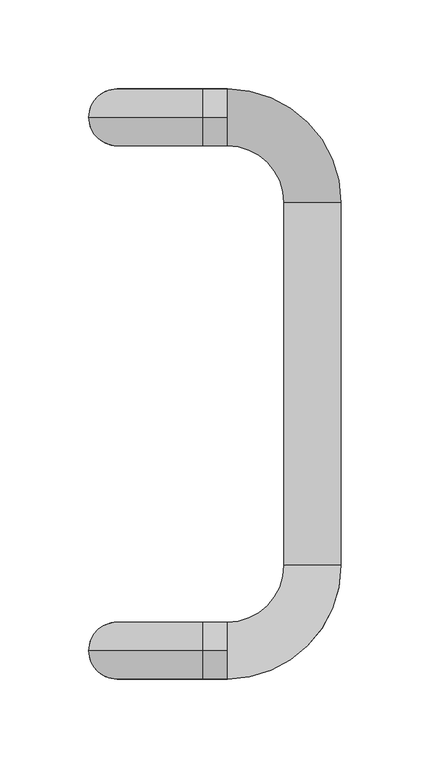
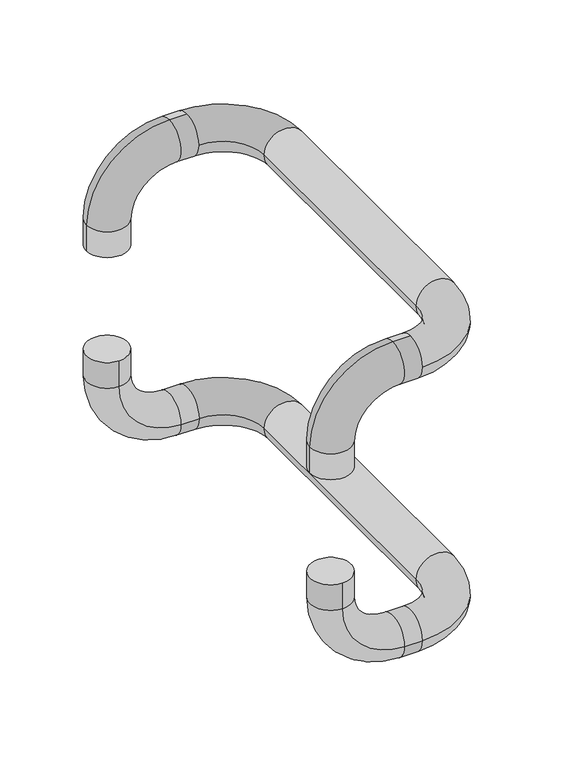
"""IFC4 building model written with IfcOpenShell, lengths in millimetres: proxy geometry, Architectural Hardware_HT7132_ASSA ABLOY_9402611AX26 : HT7132_9402611AX26."""

from ifc_helpers import new_model, si_unit, point, frame, origin, place, context, project, spatial, circle_curve, ellipse_curve, trimmed, source, transform, mapped, element, save
from ifc_brep_helpers import plane_surface, cylinder_surface, revolved_surface, advanced_brep


def specialty_equipment_07a0182d(model_context):
    return source(origin(), model_context, "Body", "AdvancedBrep", [
        advanced_brep(
        [(0.0, 166.0, -86.0), (0.0, 134.0, -86.0), (0.0, 134.0, -107.0), (0.0, 166.0, -107.0), (48.0, 134.0, -155.0), (48.0, 166.0, -155.0), (62.0, 134.0, -155.0), (62.0, 166.0, -155.0), (94.0, -102.0, -155.0), (126.0, -102.0, -155.0), (62.0, -166.0, -155.0), (62.0, -134.0, -155.0), (94.0, 102.0, -155.0), (126.0, 102.0, -155.0), (0.0, -166.0, -86.0), (0.0, -134.0, -86.0), (0.0, -166.0, -107.0), (0.0, -134.0, -107.0), (48.0, -166.0, -155.0), (48.0, -134.0, -155.0)],
        [
            (0, 1, circle_curve(frame((0.0, 150.0, -86.0), z_axis=(0.0, 0.0, 1.0), x_axis=(0.0, -1.0, 0.0)), 16.0)),
            (1, 0, circle_curve(frame((0.0, 150.0, -86.0), z_axis=(0.0, 0.0, 1.0), x_axis=(0.0, -1.0, 0.0)), 16.0)),
            (1, 2),
            (2, 3, circle_curve(frame((0.0, 150.0, -107.0), z_axis=(0.0, 0.0, 1.0), x_axis=(0.0, -1.0, 0.0)), 16.0)),
            (3, 0),
            (3, 2, circle_curve(frame((0.0, 150.0, -107.0), z_axis=(0.0, 0.0, 1.0), x_axis=(0.0, -1.0, 0.0)), 16.0)),
            (2, 4, circle_curve(frame((48.0, 134.0, -107.0), z_axis=(0.0, -1.0, 0.0), x_axis=(-1.0, 0.0, 0.0)), 48.0)),
            (4, 5, circle_curve(frame((48.0, 150.0, -155.0), z_axis=(-1.0, 0.0, 0.0), x_axis=(0.0, -1.0, 0.0)), 16.0)),
            (5, 3, circle_curve(frame((48.0, 166.0, -107.0), z_axis=(0.0, 1.0, 0.0), x_axis=(-1.0, 0.0, 0.0)), 48.0)),
            (5, 4, circle_curve(frame((48.0, 150.0, -155.0), z_axis=(-1.0, 0.0, 0.0), x_axis=(0.0, -1.0, 0.0)), 16.0)),
            (4, 6),
            (6, 7, circle_curve(frame((62.0, 150.0, -155.0), z_axis=(-1.0, 0.0, 0.0), x_axis=(0.0, -1.0, 0.0)), 16.0)),
            (7, 5),
            (7, 6, circle_curve(frame((62.0, 150.0, -155.0), z_axis=(-1.0, 0.0, 0.0), x_axis=(0.0, -1.0, 0.0)), 16.0)),
            (8, 9, circle_curve(frame((110.0, -102.0, -155.0), z_axis=(0.0, -1.0, 0.0), x_axis=(1.0, 0.0, 0.0)), 16.0)),
            (9, 10, circle_curve(frame((62.0, -102.0, -155.0), z_axis=(0.0, 0.0, -1.0), x_axis=(0.0, -1.0, 0.0)), 64.0)),
            (10, 11, circle_curve(frame((62.0, -150.0, -155.0), z_axis=(1.0, 0.0, 0.0), x_axis=(0.0, -1.0, 0.0)), 16.0)),
            (11, 8, circle_curve(frame((62.0, -102.0, -155.0), z_axis=(0.0, 0.0, 1.0), x_axis=(0.0, -1.0, 0.0)), 32.0)),
            (11, 10, circle_curve(frame((62.0, -150.0, -155.0), z_axis=(1.0, 0.0, 0.0), x_axis=(0.0, -1.0, 0.0)), 16.0)),
            (9, 8, circle_curve(frame((110.0, -102.0, -155.0), z_axis=(0.0, -1.0, 0.0), x_axis=(1.0, 0.0, 0.0)), 16.0)),
            (8, 12),
            (12, 13, circle_curve(frame((110.0, 102.0, -155.0), z_axis=(0.0, -1.0, 0.0), x_axis=(1.0, 0.0, 0.0)), 16.0)),
            (13, 9),
            (13, 12, circle_curve(frame((110.0, 102.0, -155.0), z_axis=(0.0, -1.0, 0.0), x_axis=(1.0, 0.0, 0.0)), 16.0)),
            (12, 6, circle_curve(frame((62.0, 102.0, -155.0), z_axis=(0.0, 0.0, 1.0), x_axis=(1.0, 0.0, 0.0)), 32.0)),
            (7, 13, circle_curve(frame((62.0, 102.0, -155.0), z_axis=(0.0, 0.0, -1.0), x_axis=(1.0, 0.0, 0.0)), 64.0)),
            (14, 15, circle_curve(frame((0.0, -150.0, -86.0), z_axis=(0.0, 0.0, 1.0), x_axis=(0.0, 1.0, 0.0)), 16.0)),
            (15, 14, circle_curve(frame((0.0, -150.0, -86.0), z_axis=(0.0, 0.0, 1.0), x_axis=(0.0, 1.0, 0.0)), 16.0)),
            (14, 16),
            (16, 17, circle_curve(frame((0.0, -150.0, -107.0), z_axis=(0.0, 0.0, 1.0), x_axis=(0.0, 1.0, 0.0)), 16.0)),
            (17, 15),
            (17, 16, circle_curve(frame((0.0, -150.0, -107.0), z_axis=(0.0, 0.0, 1.0), x_axis=(0.0, 1.0, 0.0)), 16.0)),
            (16, 18, circle_curve(frame((48.0, -166.0, -107.0), z_axis=(0.0, -1.0, 0.0), x_axis=(-1.0, 0.0, 0.0)), 48.0)),
            (18, 19, circle_curve(frame((48.0, -150.0, -155.0), z_axis=(-1.0, 0.0, 0.0), x_axis=(0.0, 1.0, 0.0)), 16.0)),
            (19, 17, circle_curve(frame((48.0, -134.0, -107.0), z_axis=(0.0, 1.0, 0.0), x_axis=(-1.0, 0.0, 0.0)), 48.0)),
            (19, 18, circle_curve(frame((48.0, -150.0, -155.0), z_axis=(-1.0, 0.0, 0.0), x_axis=(0.0, 1.0, 0.0)), 16.0)),
            (18, 10),
            (11, 19),
        ],
        [
            plane_surface(frame((0.0, 0.0, -86.0), z_axis=(0.0, 0.0, 1.0), x_axis=(0.0, -1.0, 0.0))),
            cylinder_surface(frame((0.0, 150.0, -86.0), z_axis=(0.0, 0.0, 1.0), x_axis=(0.0, -1.0, 0.0)), 16.0),
            revolved_surface(trimmed(ellipse_curve(frame((0.0, 150.0, -107.0), z_axis=(0.0, 0.0, -1.0), x_axis=(0.0, -1.0, 0.0)), 16.0, 16.0), [point((0.0, 166.0, -107.0))], [point((0.0, 134.0, -107.0))], True, "CARTESIAN"), (48.0, 0.0, -107.0), (0.0, 1.0, 0.0)),
            revolved_surface(trimmed(ellipse_curve(frame((0.0, 150.0, -107.0), z_axis=(0.0, 0.0, -1.0), x_axis=(0.0, -1.0, 0.0)), 16.0, 16.0), [point((0.0, 134.0, -107.0))], [point((0.0, 166.0, -107.0))], True, "CARTESIAN"), (48.0, 0.0, -107.0), (0.0, 1.0, 0.0)),
            cylinder_surface(frame((48.0, 150.0, -155.0), z_axis=(-1.0, 0.0, 0.0), x_axis=(0.0, -1.0, 0.0)), 16.0),
            revolved_surface(trimmed(ellipse_curve(frame((62.0, -150.0, -155.0), z_axis=(1.0, 0.0, 0.0), x_axis=(0.0, -1.0, 0.0)), 16.0, 16.0), [point((62.0, -166.0, -155.0))], [point((62.0, -134.0, -155.0))], True, "CARTESIAN"), (62.0, -102.0, -86.0), (0.0, 0.0, -1.0)),
            revolved_surface(trimmed(ellipse_curve(frame((62.0, -150.0, -155.0), z_axis=(1.0, 0.0, 0.0), x_axis=(0.0, -1.0, 0.0)), 16.0, 16.0), [point((62.0, -134.0, -155.0))], [point((62.0, -166.0, -155.0))], True, "CARTESIAN"), (62.0, -102.0, -86.0), (0.0, 0.0, -1.0)),
            cylinder_surface(frame((110.0, -102.0, -155.0), z_axis=(0.0, -1.0, 0.0), x_axis=(1.0, 0.0, 0.0)), 16.0),
            revolved_surface(trimmed(ellipse_curve(frame((110.0, 102.0, -155.0), z_axis=(0.0, 1.0, 0.0), x_axis=(1.0, 0.0, 0.0)), 16.0, 16.0), [point((126.0, 102.0, -155.0))], [point((94.0, 102.0, -155.0))], True, "CARTESIAN"), (62.0, 102.0, -86.0), (0.0, 0.0, -1.0)),
            revolved_surface(trimmed(ellipse_curve(frame((110.0, 102.0, -155.0), z_axis=(0.0, 1.0, 0.0), x_axis=(1.0, 0.0, 0.0)), 16.0, 16.0), [point((94.0, 102.0, -155.0))], [point((126.0, 102.0, -155.0))], True, "CARTESIAN"), (62.0, 102.0, -86.0), (0.0, 0.0, -1.0)),
            plane_surface(frame((0.0, 0.0, -86.0), z_axis=(0.0, 0.0, 1.0), x_axis=(0.0, 1.0, 0.0))),
            cylinder_surface(frame((0.0, -150.0, -86.0), z_axis=(0.0, 0.0, 1.0), x_axis=(0.0, 1.0, 0.0)), 16.0),
            revolved_surface(trimmed(ellipse_curve(frame((0.0, -150.0, -107.0), z_axis=(0.0, 0.0, -1.0), x_axis=(0.0, 1.0, 0.0)), 16.0, 16.0), [point((0.0, -134.0, -107.0))], [point((0.0, -166.0, -107.0))], True, "CARTESIAN"), (48.0, 0.0, -107.0), (0.0, 1.0, 0.0)),
            revolved_surface(trimmed(ellipse_curve(frame((0.0, -150.0, -107.0), z_axis=(0.0, 0.0, -1.0), x_axis=(0.0, 1.0, 0.0)), 16.0, 16.0), [point((0.0, -166.0, -107.0))], [point((0.0, -134.0, -107.0))], True, "CARTESIAN"), (48.0, 0.0, -107.0), (0.0, 1.0, 0.0)),
            cylinder_surface(frame((48.0, -150.0, -155.0), z_axis=(-1.0, 0.0, 0.0), x_axis=(0.0, 1.0, 0.0)), 16.0),
        ],
        [
            (0, [[1, 2]]),
            (1, [[3, 4, 5, -2]]),
            (1, [[-5, 6, -3, -1]]),
            (2, [[7, 8, 9, -4]]),
            (3, [[-9, 10, -7, -6]]),
            (4, [[11, 12, 13, -8]]),
            (4, [[-13, 14, -11, -10]]),
            (5, [[15, 16, 17, 18]]),
            (6, [[19, -16, 20, -18]]),
            (7, [[21, 22, 23, -15]]),
            (7, [[-23, 24, -21, -20]]),
            (8, [[25, -14, 26, -22]]),
            (9, [[-26, -12, -25, -24]]),
            (10, [[27, 28]]),
            (11, [[29, 30, 31, -27]]),
            (11, [[-31, 32, -29, -28]]),
            (12, [[33, 34, 35, -30]]),
            (13, [[-35, 36, -33, -32]]),
            (14, [[37, -19, 38, -34]]),
            (14, [[-38, -17, -37, -36]]),
        ],
    ),
        advanced_brep(
        [(94.0, -102.0, 69.0), (126.0, -102.0, 69.0), (62.0, -166.0, 69.0), (62.0, -150.0, 53.0), (62.0, -134.0, 69.0), (62.0, -150.0, 85.0), (94.0, 102.0, 69.0), (126.0, 102.0, 69.0), (62.0, 134.0, 69.0), (62.0, 150.0, 53.0), (62.0, 166.0, 69.0), (62.0, 150.0, 85.0), (-16.0, -150.0, 0.0), (16.0, -150.0, 0.0), (16.0, -150.0, 21.0), (-16.0, -150.0, 21.0), (48.0, -150.0, 53.0), (48.0, -150.0, 85.0), (-16.0, 150.0, 0.0), (16.0, 150.0, 0.0), (-16.0, 150.0, 21.0), (16.0, 150.0, 21.0), (48.0, 150.0, 85.0), (48.0, 150.0, 53.0)],
        [
            (0, 1, circle_curve(frame((110.0, -102.0, 69.0), z_axis=(0.0, -1.0, 0.0), x_axis=(-1.0, 0.0, 0.0)), 16.0)),
            (1, 2, circle_curve(frame((62.0, -102.0, 69.0), z_axis=(0.0, 0.0, -1.0), x_axis=(0.0, -1.0, 0.0)), 64.0)),
            (2, 3, circle_curve(frame((62.0, -150.0, 69.0), z_axis=(1.0, 0.0, 0.0), x_axis=(0.0, 1.0, 0.0)), 16.0)),
            (3, 4, circle_curve(frame((62.0, -150.0, 69.0), z_axis=(1.0, 0.0, 0.0), x_axis=(0.0, 1.0, 0.0)), 16.0)),
            (4, 0, circle_curve(frame((62.0, -102.0, 69.0), z_axis=(0.0, 0.0, 1.0), x_axis=(0.0, -1.0, 0.0)), 32.0)),
            (4, 5, circle_curve(frame((62.0, -150.0, 69.0), z_axis=(1.0, 0.0, 0.0), x_axis=(0.0, 1.0, 0.0)), 16.0)),
            (5, 2, circle_curve(frame((62.0, -150.0, 69.0), z_axis=(1.0, 0.0, 0.0), x_axis=(0.0, 1.0, 0.0)), 16.0)),
            (1, 0, circle_curve(frame((110.0, -102.0, 69.0), z_axis=(0.0, -1.0, 0.0), x_axis=(-1.0, 0.0, 0.0)), 16.0)),
            (0, 6),
            (6, 7, circle_curve(frame((110.0, 102.0, 69.0), z_axis=(0.0, -1.0, 0.0), x_axis=(-1.0, 0.0, 0.0)), 16.0)),
            (7, 1),
            (7, 6, circle_curve(frame((110.0, 102.0, 69.0), z_axis=(0.0, -1.0, 0.0), x_axis=(-1.0, 0.0, 0.0)), 16.0)),
            (6, 8, circle_curve(frame((62.0, 102.0, 69.0), z_axis=(0.0, 0.0, 1.0), x_axis=(1.0, 0.0, 0.0)), 32.0)),
            (8, 9, circle_curve(frame((62.0, 150.0, 69.0), z_axis=(1.0, 0.0, 0.0), x_axis=(0.0, -1.0, 0.0)), 16.0)),
            (9, 10, circle_curve(frame((62.0, 150.0, 69.0), z_axis=(1.0, 0.0, 0.0), x_axis=(0.0, -1.0, 0.0)), 16.0)),
            (10, 7, circle_curve(frame((62.0, 102.0, 69.0), z_axis=(0.0, 0.0, -1.0), x_axis=(1.0, 0.0, 0.0)), 64.0)),
            (10, 11, circle_curve(frame((62.0, 150.0, 69.0), z_axis=(1.0, 0.0, 0.0), x_axis=(0.0, -1.0, 0.0)), 16.0)),
            (11, 8, circle_curve(frame((62.0, 150.0, 69.0), z_axis=(1.0, 0.0, 0.0), x_axis=(0.0, -1.0, 0.0)), 16.0)),
            (12, 13, circle_curve(frame((0.0, -150.0, 0.0), z_axis=(0.0, 0.0, -1.0), x_axis=(1.0, 0.0, 0.0)), 16.0)),
            (13, 12, circle_curve(frame((0.0, -150.0, 0.0), z_axis=(0.0, 0.0, -1.0), x_axis=(1.0, 0.0, 0.0)), 16.0)),
            (13, 14),
            (14, 15, circle_curve(frame((0.0, -150.0, 21.0), z_axis=(0.0, 0.0, -1.0), x_axis=(1.0, 0.0, 0.0)), 16.0)),
            (15, 12),
            (15, 14, circle_curve(frame((0.0, -150.0, 21.0), z_axis=(0.0, 0.0, -1.0), x_axis=(1.0, 0.0, 0.0)), 16.0)),
            (14, 16, circle_curve(frame((48.0, -150.0, 21.0), z_axis=(0.0, 1.0, 0.0), x_axis=(-1.0, 0.0, 0.0)), 32.0)),
            (16, 17, circle_curve(frame((48.0, -150.0, 69.0), z_axis=(-1.0, 0.0, 0.0), x_axis=(0.0, 0.0, -1.0)), 16.0)),
            (17, 15, circle_curve(frame((48.0, -150.0, 21.0), z_axis=(0.0, -1.0, 0.0), x_axis=(-1.0, 0.0, 0.0)), 64.0)),
            (17, 16, circle_curve(frame((48.0, -150.0, 69.0), z_axis=(-1.0, 0.0, 0.0), x_axis=(0.0, 0.0, -1.0)), 16.0)),
            (16, 3),
            (5, 17),
            (18, 19, circle_curve(frame((0.0, 150.0, 0.0), z_axis=(0.0, 0.0, -1.0), x_axis=(1.0, 0.0, 0.0)), 16.0)),
            (19, 18, circle_curve(frame((0.0, 150.0, 0.0), z_axis=(0.0, 0.0, -1.0), x_axis=(1.0, 0.0, 0.0)), 16.0)),
            (18, 20),
            (20, 21, circle_curve(frame((0.0, 150.0, 21.0), z_axis=(0.0, 0.0, -1.0), x_axis=(1.0, 0.0, 0.0)), 16.0)),
            (21, 19),
            (21, 20, circle_curve(frame((0.0, 150.0, 21.0), z_axis=(0.0, 0.0, -1.0), x_axis=(1.0, 0.0, 0.0)), 16.0)),
            (20, 22, circle_curve(frame((48.0, 150.0, 21.0), z_axis=(0.0, 1.0, 0.0), x_axis=(-1.0, 0.0, 0.0)), 64.0)),
            (22, 23, circle_curve(frame((48.0, 150.0, 69.0), z_axis=(-1.0, 0.0, 0.0), x_axis=(0.0, 0.0, -1.0)), 16.0)),
            (23, 21, circle_curve(frame((48.0, 150.0, 21.0), z_axis=(0.0, -1.0, 0.0), x_axis=(-1.0, 0.0, 0.0)), 32.0)),
            (23, 22, circle_curve(frame((48.0, 150.0, 69.0), z_axis=(-1.0, 0.0, 0.0), x_axis=(0.0, 0.0, -1.0)), 16.0)),
            (22, 11),
            (9, 23),
        ],
        [
            revolved_surface(trimmed(ellipse_curve(frame((62.0, -150.0, 69.0), z_axis=(1.0, 0.0, 0.0), x_axis=(0.0, 1.0, 0.0)), 16.0, 16.0), [point((62.0, -166.0, 69.0))], [point((62.0, -134.0, 69.0))], True, "CARTESIAN"), (62.0, -102.0, 0.0), (0.0, 0.0, -1.0)),
            revolved_surface(trimmed(ellipse_curve(frame((62.0, -150.0, 69.0), z_axis=(1.0, 0.0, 0.0), x_axis=(0.0, 1.0, 0.0)), 16.0, 16.0), [point((62.0, -134.0, 69.0))], [point((62.0, -166.0, 69.0))], True, "CARTESIAN"), (62.0, -102.0, 0.0), (0.0, 0.0, -1.0)),
            cylinder_surface(frame((110.0, -102.0, 69.0), z_axis=(0.0, -1.0, 0.0), x_axis=(-1.0, 0.0, 0.0)), 16.0),
            revolved_surface(trimmed(ellipse_curve(frame((110.0, 102.0, 69.0), z_axis=(0.0, 1.0, 0.0), x_axis=(-1.0, 0.0, 0.0)), 16.0, 16.0), [point((126.0, 102.0, 69.0))], [point((94.0, 102.0, 69.0))], True, "CARTESIAN"), (62.0, 102.0, 0.0), (0.0, 0.0, -1.0)),
            revolved_surface(trimmed(ellipse_curve(frame((110.0, 102.0, 69.0), z_axis=(0.0, 1.0, 0.0), x_axis=(-1.0, 0.0, 0.0)), 16.0, 16.0), [point((94.0, 102.0, 69.0))], [point((126.0, 102.0, 69.0))], True, "CARTESIAN"), (62.0, 102.0, 0.0), (0.0, 0.0, -1.0)),
            plane_surface(frame((0.0, 0.0, 0.0), z_axis=(0.0, 0.0, -1.0), x_axis=(0.0, 1.0, 0.0))),
            cylinder_surface(frame((0.0, -150.0, 0.0), z_axis=(0.0, 0.0, -1.0), x_axis=(1.0, 0.0, 0.0)), 16.0),
            revolved_surface(trimmed(ellipse_curve(frame((0.0, -150.0, 21.0), z_axis=(0.0, 0.0, 1.0), x_axis=(1.0, 0.0, 0.0)), 16.0, 16.0), [point((-16.0, -150.0, 21.0))], [point((16.0, -150.0, 21.0))], True, "CARTESIAN"), (48.0, 0.0, 21.0), (0.0, -1.0, 0.0)),
            revolved_surface(trimmed(ellipse_curve(frame((0.0, -150.0, 21.0), z_axis=(0.0, 0.0, 1.0), x_axis=(1.0, 0.0, 0.0)), 16.0, 16.0), [point((16.0, -150.0, 21.0))], [point((-16.0, -150.0, 21.0))], True, "CARTESIAN"), (48.0, 0.0, 21.0), (0.0, -1.0, 0.0)),
            cylinder_surface(frame((48.0, -150.0, 69.0), z_axis=(-1.0, 0.0, 0.0), x_axis=(0.0, 0.0, -1.0)), 16.0),
            plane_surface(frame((0.0, 0.0, 0.0), z_axis=(0.0, 0.0, -1.0), x_axis=(0.0, -1.0, 0.0))),
            cylinder_surface(frame((0.0, 150.0, 0.0), z_axis=(0.0, 0.0, -1.0), x_axis=(1.0, 0.0, 0.0)), 16.0),
            revolved_surface(trimmed(ellipse_curve(frame((0.0, 150.0, 21.0), z_axis=(0.0, 0.0, 1.0), x_axis=(1.0, 0.0, 0.0)), 16.0, 16.0), [point((16.0, 150.0, 21.0))], [point((-16.0, 150.0, 21.0))], True, "CARTESIAN"), (48.0, 0.0, 21.0), (0.0, -1.0, 0.0)),
            revolved_surface(trimmed(ellipse_curve(frame((0.0, 150.0, 21.0), z_axis=(0.0, 0.0, 1.0), x_axis=(1.0, 0.0, 0.0)), 16.0, 16.0), [point((-16.0, 150.0, 21.0))], [point((16.0, 150.0, 21.0))], True, "CARTESIAN"), (48.0, 0.0, 21.0), (0.0, -1.0, 0.0)),
            cylinder_surface(frame((48.0, 150.0, 69.0), z_axis=(-1.0, 0.0, 0.0), x_axis=(0.0, 0.0, -1.0)), 16.0),
        ],
        [
            (0, [[1, 2, 3, 4, 5]]),
            (1, [[6, 7, -2, 8, -5]]),
            (2, [[9, 10, 11, -1]]),
            (2, [[-11, 12, -9, -8]]),
            (3, [[13, 14, 15, 16, -10]]),
            (4, [[-16, 17, 18, -13, -12]]),
            (5, [[19, 20]]),
            (6, [[21, 22, 23, -20]]),
            (6, [[-23, 24, -21, -19]]),
            (7, [[25, 26, 27, -22]]),
            (8, [[-27, 28, -25, -24]]),
            (9, [[29, -3, -7, 30, -26]]),
            (9, [[-30, -6, -4, -29, -28]]),
            (10, [[31, 32]]),
            (11, [[33, 34, 35, -31]]),
            (11, [[-35, 36, -33, -32]]),
            (12, [[37, 38, 39, -34]]),
            (13, [[-39, 40, -37, -36]]),
            (14, [[41, -17, -15, 42, -38]]),
            (14, [[-42, -14, -18, -41, -40]]),
        ],
    ),
    ])


if __name__ == "__main__":
    model = new_model("IFC4")
    model_context = context("Model", 3, world=origin())
    ifc_project = project(units=[si_unit("LENGTHUNIT", "METRE", prefix="MILLI")], contexts=[model_context])
    site = spatial("IfcSite", under=ifc_project)
    building = spatial("IfcBuilding", under=site)
    placement = place(None, origin())
    specialty_equipment_shape = specialty_equipment_07a0182d(model_context)
    element("IfcBuildingElementProxy", 1, Name="Architectural Hardware_HT7132_ASSA ABLOY_9402611AX26 : HT7132_9402611AX26", ObjectType="Architectural Hardware_HT7132_ASSA ABLOY_9402611AX26 : HT7132_9402611AX26", at=placement, inside=building, context=model_context, shape_type="MappedRepresentation", body=[
        mapped(specialty_equipment_shape, transform((0.0, 0.0, 0.0), x_axis=(1.0, 0.0, 0.0), y_axis=(0.0, 1.0, 0.0), z_axis=(0.0, 0.0, 1.0))),
    ])
    save(model, "model.ifc")

# Revit data of these elements
# Type "Architectural Hardware_HT7132_ASSA ABLOY_9402611AX26 : HT7132_9402611AX26"
#   Uniclass 2.0 Description = "Door Hardware Systems"
#   Uniclass 2.0 Code = "SS-25-38-20-20"
#   Uniclass 1.4 Description = "Door furniture"
#   Uniclass 1.4 Code = "L4181"
#   URL = "http://assaabloyopeningsolutions.no/prosjekt"
#   UNSPSC Code = ""
#   Type Comments = "HT7132"
#   Region Europe = "NO"
#   Reference Standards = "NS-EN 1906"
#   Provider = "ASSA ABLOY Opening Solutions Norway"
#   Product Range = "TrioVing Line"
#   Product Guid = "be3695cd-0f10-4d8b-9704-0e65f31cb4bc"
#   Product Group = "Architectural and Accessory Hardware"
#   Product Datasheet = "http://xnet.trioving.be/Katalog.asp?ProdId=115479"
#   OmniClass Description = "Door Accessories"
#   OmniClass Code = "23-17 11 11 25"
#   Name = "HT7132"
#   NBS Reference Description = "Door Hardware Systems"
#   NBS Reference Code = "25-38-20-20"
#   Model = "Architectural Hardware_HT7132_ASSA ABLOY_9402611AX26"
#   Manufacturer = "ASSA ABLOY"
#   ISO = "ISO 14001"
#   IFC Classification = "Door"
#   Environmental Product Declaration (EPD) = ""
#   Description = "Push Pull Bent 300mm Ø32mm"
#   Date of publishing = "2015-11-16"
#   Contact Provider = "http://assaabloyopeningsolutions.no/prosjekt"
#   BIMobject category = "Door Hardware"
#   BIMobject Unique ref = "9402611AX26"
#   BIMobject Instructions Video = "https://www.youtube.com/user/BIMobject"
#   BIMobject Brand = "ASSA ABLOY NO"
#   Article Number = "9402611AX26"
#   Accessories = ""
#   Panel Thickness [instance default] = 0' - 3.38583"
#   Offset Perpendicular [instance default] = 2' - 7.4929"
#   Offset Horizontal [instance default] = 1' - 11.29337"
#   Handle Offset [instance default] = 0' - 1.9685"
#   Edition number = 2
#   Finish = Stainless Steel
#   Default Elevation = 0
#   Cost = 0
# Element 1 (IfcBuildingElementProxy, "Architectural Hardware_HT7132_ASSA ABLOY_9402611AX26 : HT7132_9402611AX26")
#   Offset Perpendicular = 3' - 2.35433"
#   Offset Horizontal = 3' - 0.58268"
#   Handle Offset = 0' - 2.26378"
#   Materials on its faces: "Stainless Steel"
# Materials
#   "Stainless Steel": class "Metal", colour RGB 0 0 0, transparency 0, Description = "Stainless Steel 18/8", Cost = 0
